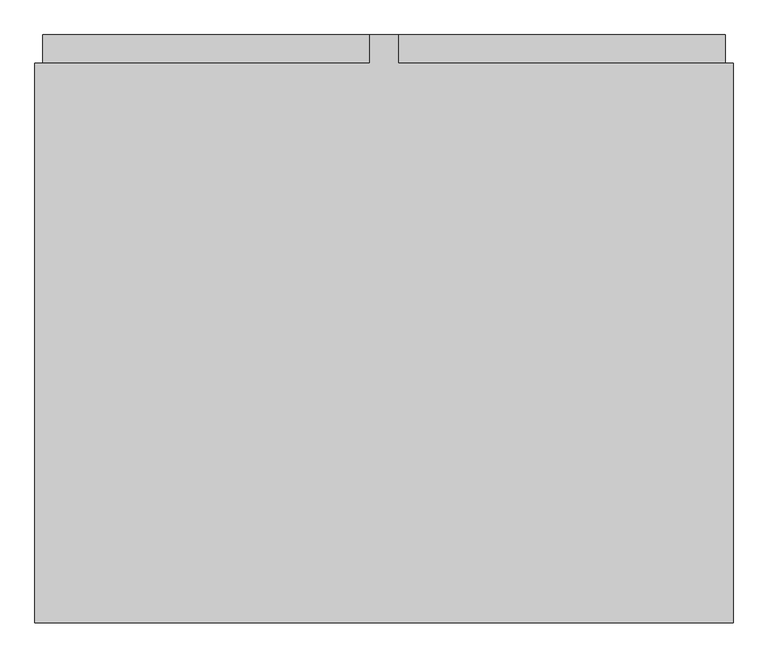
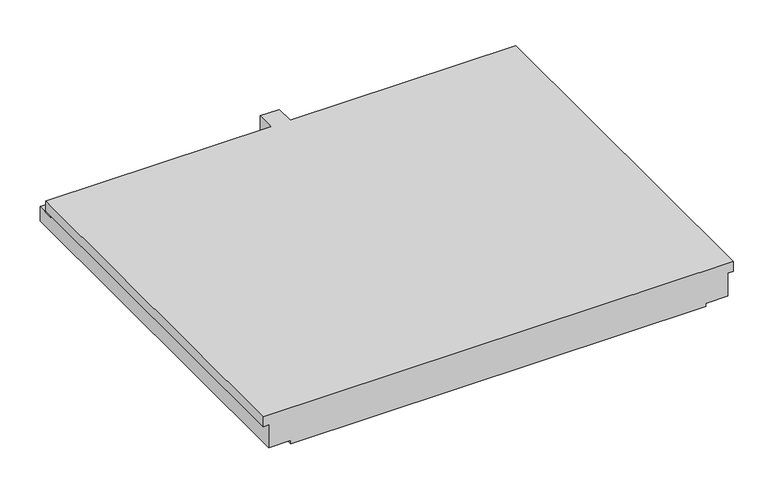
"""IFC4 building model written with IfcOpenShell, lengths in millimetres: proxy geometry, NLRS_24_GM_UN_rechthoekig bordes prefab-AV_gen_rsf : prefab bordes_gen__2300x2730."""

from ifc_helpers import new_model, si_unit, origin, place, context, project, spatial, faceted_brep, source, transform, mapped, element, save


def generic_models_39f13373(model_context):
    return source(origin(), model_context, "Body", "Brep", [
        faceted_brep([(1365.0, 2190.0, 0.0), (1365.0, 0.0, 0.0), (1365.0, 0.0, -60.0), (1365.0, 2190.0, -60.0), (55.0, 2300.0, -110.0), (55.0, 2190.0, -110.0), (1335.0, 2190.0, -110.0), (1335.0, 2300.0, -110.0), (55.0, 2190.0, 0.0), (1335.0, 2190.0, -60.0), (55.0, 2300.0, 0.0), (-55.0, 2300.0, 0.0), (-55.0, 2300.0, -110.0), (-55.0, 2190.0, -110.0), (-55.0, 2190.0, 0.0), (-1365.0, 0.0, 0.0), (-1365.0, 2190.0, 0.0), (-1365.0, 2190.0, -60.0), (-1365.0, 0.0, -60.0), (-1335.0, 2300.0, -110.0), (1335.0, 2300.0, -200.0), (1205.0, 2300.0, -200.0), (1205.0, 2300.0, -220.0), (-1205.0, 2300.0, -220.0), (-1205.0, 2300.0, -200.0), (-1335.0, 2300.0, -200.0), (-1335.0, 2190.0, -110.0), (-1335.0, 2190.0, -60.0), (-1335.0, 0.0, -60.0), (-1335.0, 0.0, -200.0), (-1205.0, 0.0, -200.0), (-1205.0, 0.0, -220.0), (1205.0, 0.0, -220.0), (1205.0, 0.0, -200.0), (1335.0, 0.0, -200.0), (1335.0, 0.0, -60.0)], [[[0, 1, 2, 3]], [[4, 5, 6, 7]], [[8, 0, 3, 9, 6, 5]], [[10, 8, 5, 4]], [[11, 12, 13, 14]], [[15, 16, 17, 18]], [[19, 12, 11, 10, 4, 7, 20, 21, 22, 23, 24, 25]], [[12, 19, 26, 13]], [[16, 14, 13, 26, 27, 17]], [[16, 15, 1, 0, 8, 10, 11, 14]], [[15, 18, 28, 29, 30, 31, 32, 33, 34, 35, 2, 1]], [[31, 23, 22, 32]], [[27, 28, 18, 17]], [[25, 29, 28, 27, 26, 19]], [[29, 25, 24, 30]], [[30, 24, 23, 31]], [[35, 9, 3, 2]], [[34, 20, 7, 6, 9, 35]], [[20, 34, 33, 21]], [[21, 33, 32, 22]]]),
    ])


if __name__ == "__main__":
    model = new_model("IFC4")
    model_context = context("Model", 3, world=origin())
    ifc_project = project(units=[si_unit("LENGTHUNIT", "METRE", prefix="MILLI")], contexts=[model_context])
    site = spatial("IfcSite", under=ifc_project)
    building = spatial("IfcBuilding", under=site)
    placement = place(None, origin())
    generic_models_shape = generic_models_39f13373(model_context)
    element("IfcBuildingElementProxy", 1, Name="NLRS_24_GM_UN_rechthoekig bordes prefab-AV_gen_rsf : prefab bordes_gen__2300x2730", ObjectType="NLRS_24_GM_UN_rechthoekig bordes prefab-AV_gen_rsf : prefab bordes_gen__2300x2730", at=placement, inside=building, context=model_context, shape_type="MappedRepresentation", body=[
        mapped(generic_models_shape, transform((0.0, 0.0, 0.0), x_axis=(1.0, 0.0, 0.0), y_axis=(0.0, 1.0, 0.0), z_axis=(0.0, 0.0, 1.0))),
    ])
    save(model, "model.ifc")

# Revit data of these elements
# Type "NLRS_24_GM_UN_rechthoekig bordes prefab-AV_gen_rsf : prefab bordes_gen__2300x2730"
#   Export Type to IFC As = "IfcStair"
#   Type IfcGUID = "2CEqVLPNH8KRN7ghwV3ZdG"
#   Type Comments = " "
#   Model = " "
#   Manufacturer = " "
#   Description = "rechthoekig bordes prefab\r\n1930x4395"
#   Assembly Code = "24.15"
#   Width = 2730 mm
#   Thickness = 220 mm
#   Perimeter = 10060 mm
#   NLRS_C_lengte_02 = 1310 mm
#   NLRS_C_lengte_01 = 1310 mm
#   NLRS_C_hoogte_02 = 110 mm
#   NLRS_C_hoogte_01 = 110 mm
#   NLRS_C_diepte_04 = 2300 mm
#   NLRS_C_diepte_03 = 2300 mm
#   NLRS_C_diepte_02 = 110 mm
#   NLRS_C_diepte_01 = 110 mm
#   Length = 2300 mm
#   Default Elevation = 1219.2 mm
#   Area = 6.279 m²
#   NLRS_C_materiaal = NLRS_f2_beton prefab_gen_rsf
#   Keynote = ""
# Element 1 (IfcBuildingElementProxy, "NLRS_24_GM_UN_rechthoekig bordes prefab-AV_gen_rsf : prefab bordes_gen__2300x2730")
#   Materials on its faces: "NLRS_f2_beton prefab_gen_rsf"
# Materials
#   "NLRS_f2_beton prefab_gen_rsf": class "F - Niet gebakken kunststeen", colour RGB 129 133 118, transparency 0, Keynote = "f2", Manufacturer = "Revit Standards Foundation", URL = "www.revitstandards.org", Description = "beton prefab", Cost = 0
